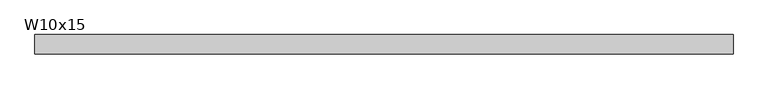
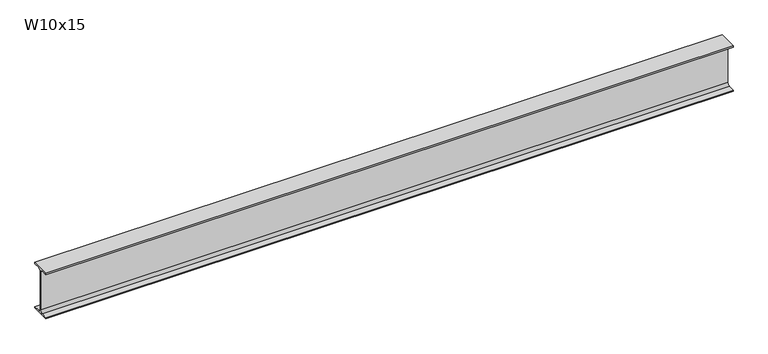
"""IFC4 building model written with IfcOpenShell, lengths in millimetres: beam geometry, RME W-Wide Flange : W10x15."""

from ifc_helpers import new_model, si_unit, point, frame, frame_2d, origin, place, context, project, spatial, polyline, circle_curve, trimmed, segment, composite_curve, outline, extrude, source, transform, mapped, element, save


def w10x15_de617878(model_context):
    return source(origin(), model_context, "Body", "SweptSolid", [
        extrude(outline(composite_curve([segment(polyline([(50.8, -120.142), (50.8, -127.0), (-50.8, -127.0), (-50.8, -120.142), (-16.7005, -120.142)]), True, "CONTINUOUS"), segment(trimmed(circle_curve(frame_2d((-16.7005, -106.3625)), 13.7795), [point((-16.7005, -120.142))], [point((-2.921, -106.3625))], True, "CARTESIAN"), True, "CONTINUOUS"), segment(polyline([(-2.921, -106.3625), (-2.921, 106.3625)]), True, "CONTINUOUS"), segment(trimmed(circle_curve(frame_2d((-16.7005, 106.3625)), 13.7795), [point((-2.921, 106.3625))], [point((-16.7005, 120.142))], True, "CARTESIAN"), True, "CONTINUOUS"), segment(polyline([(-16.7005, 120.142), (-50.8, 120.142), (-50.8, 127.0), (50.8, 127.0), (50.8, 120.142), (16.7005, 120.142)]), True, "CONTINUOUS"), segment(trimmed(circle_curve(frame_2d((16.7005, 106.3625)), 13.7795), [point((16.7005, 120.142))], [point((2.921, 106.3625))], True, "CARTESIAN"), True, "CONTINUOUS"), segment(polyline([(2.921, 106.3625), (2.921, -106.3625)]), True, "CONTINUOUS"), segment(trimmed(circle_curve(frame_2d((16.7005, -106.3625)), 13.7795), [point((2.921, -106.3625))], [point((16.7005, -120.142))], True, "CARTESIAN"), True, "CONTINUOUS"), segment(polyline([(16.7005, -120.142), (50.8, -120.142)]), True, "CONTINUOUS")], self_intersect=False)), frame((-1819.9459912, 0.0, 0.0), z_axis=(1.0, 0.0, 0.0), x_axis=(0.0, 1.0, 0.0)), (0.0, 0.0, 1.0), 3642.1363586),
    ])


if __name__ == "__main__":
    model = new_model("IFC4")
    model_context = context("Model", 3, world=origin())
    ifc_project = project(units=[si_unit("LENGTHUNIT", "METRE", prefix="MILLI")], contexts=[model_context])
    site = spatial("IfcSite", under=ifc_project)
    building = spatial("IfcBuilding", under=site)
    placement = place(None, origin())
    w10x15_shape = w10x15_de617878(model_context)
    element("IfcBeam", 1, ObjectType="RME W-Wide Flange : W10x15", at=placement, inside=building, context=model_context, shape_type="MappedRepresentation", body=[
        mapped(w10x15_shape, transform((0.0, 0.0, 0.0), x_axis=(1.0, 0.0, 0.0), y_axis=(0.0, 1.0, 0.0), z_axis=(0.0, 0.0, 1.0))),
    ])
    save(model, "model.ifc")

# Revit data of these elements
# Type "RME W-Wide Flange : W10x15"
#   WELD P [instance default] = ""
#   WELD LE [instance default] = ""
#   WELD D [instance default] = ""
#   TOP SECTION SIZE [instance default] = ""
#   TOP SECTION LENGTH [instance default] = ""
#   REMARKS [instance default] = ""
#   REINF TYPE [instance default] = ""
#   Nominal Size = "W24"
#   End Bearing Capacity [instance default] = ""
#   BOT SECTION SIZE [instance default] = ""
#   BOT SECTION LENGTH [instance default] = ""
#   Assembly Code = "B10"
#   W = 15
#   Start Extension Calculation [instance default] = 10' - 0"
#   Start Extension [instance default] = -0' - 0 1/2"
#   End Extension Calculation [instance default] = 10' - 0"
#   End Extension [instance default] = -0' - 0 1/2"
#   Length [instance default] = 5' - 0"
#   bf = 0' - 4"
#   d = 0' - 10"
#   k = 0' - 0 13/16"
#   k2 = 0' - 0.5425"
#   tf = 0' - 0.27"
#   tw = 0' - 0.23"
#   A = 0.030625 SF
#   Structural Material [instance default] = Metal - Steel - ASTM A992
# Element 1 (IfcBeam, "RME W-Wide Flange : W10x15")
#   Length = 12' - 7.96711"
#   Materials on its faces: "Metal - Steel - ASTM A992"
# Materials
#   "Metal - Steel - ASTM A992": class "Metal", colour RGB 255 128 0, transparency 0
